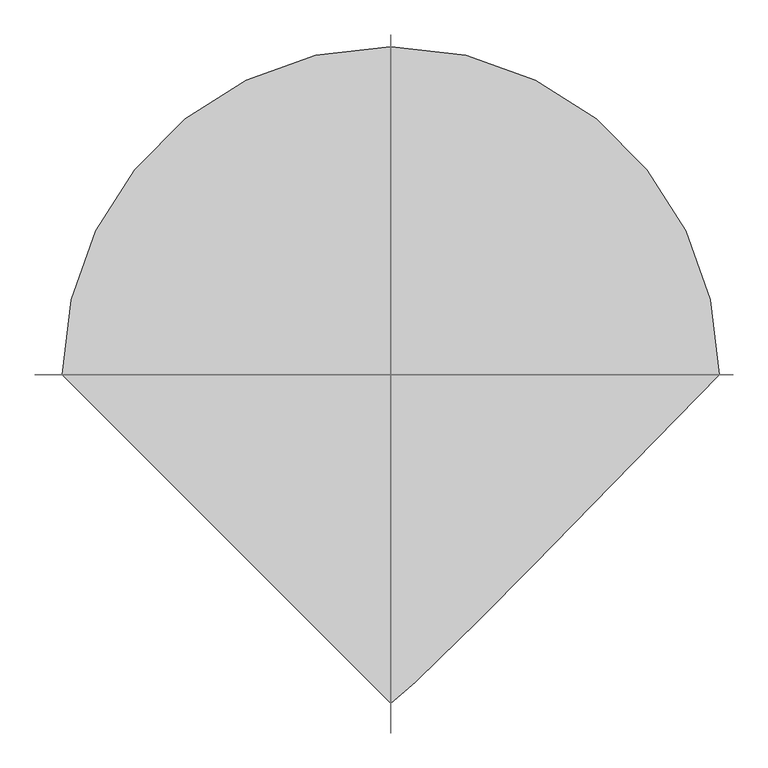
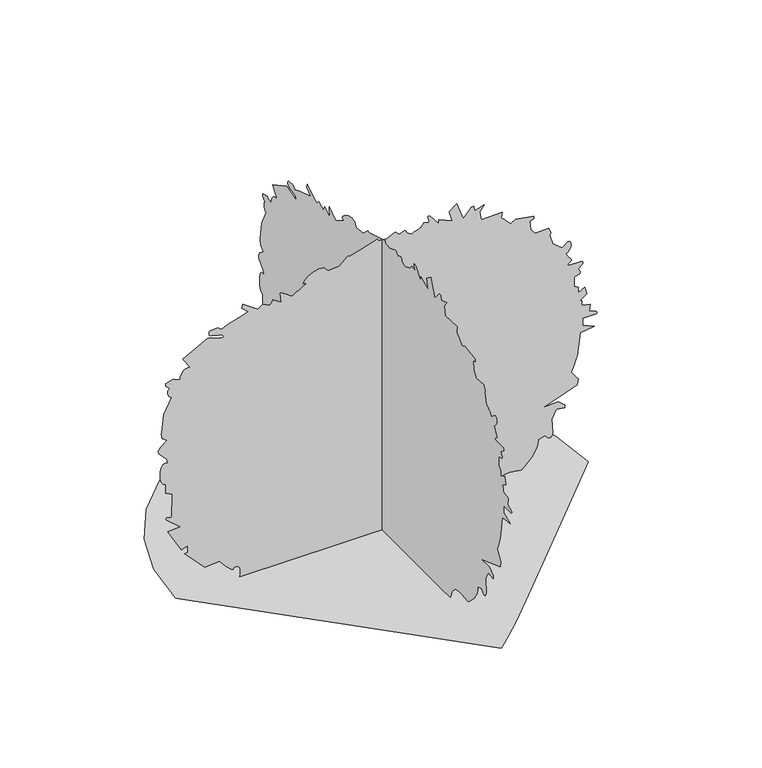
"""IFC4 building model written with IfcOpenShell, lengths in millimetres: proxy geometry, holly 26751 : holly 26751."""

from ifc_helpers import new_model, si_unit, origin, place, context, project, spatial, triangles, source, transform, mapped, element, save


def entourage_04c35473(model_context):
    return source(origin(), model_context, "Body", "Tessellation", [
        triangles([(-823.0310858, 0.0, 7.21e-05), (-801.2709314, 188.5840741, 7.21e-05), (-739.3050917, 361.7670897, 7.21e-05), (-642.0891506, 514.5912643, 7.21e-05), (-514.5912643, 642.0891506, 7.21e-05), (-361.7670897, 739.3050917, 7.21e-05), (-188.5840741, 801.2709314, 7.21e-05), (3.6e-05, 823.0310858, 7.21e-05), (188.5840741, 801.2709314, 7.21e-05), (361.7670897, 739.3050917, 7.21e-05), (514.5912643, 642.0891506, 7.21e-05), (642.0891506, 514.5912643, 7.21e-05), (739.3050917, 361.7670897, 7.21e-05), (801.2709314, 188.5838197, 7.21e-05), (823.0310858, -7.2e-05, 7.21e-05), (555.5640178, -274.3555465, 7.21e-05), (357.2763754, -476.3515926, 7.21e-05), (216.6411551, -618.0454874, 7.21e-05), (122.1254853, -711.5022102, 7.21e-05), (62.2002777, -768.7766939, 7.21e-05), (25.3349997, -801.933827, 7.21e-05), (-0.0001079, -823.0310858, 7.21e-05), (0.0, -364.688096, 1198.1839863), (0.0, -394.9268025, 1235.9816792), (0.0, -406.2653546, 1235.9816792), (0.0, -410.0448841, 1217.0841408), (0.0, -447.8426133, 1228.4226929), (0.0, -428.9450386, 1205.7430452), (0.0, -436.5040612, 1167.9452797), (0.0, -519.6585786, 1171.727389), (0.0, -515.8790491, 1149.0476686), (0.0, -517.7484844, 1147.6176687), (0.0, -521.9039357, 1143.7644882), (0.0, -527.6798913, 1138.1510954), (0.0, -534.4109121, 1131.4328281), (0.0, -541.4314502, 1124.2699659), (0.0, -548.0735593, 1117.3230789), (0.0, -553.6768147, 1111.2499758), (0.0, -572.5743894, 1122.5885279), (0.0, -644.390391, 1111.2499758), (0.0, -644.390391, 1099.9114237), (0.0, -629.2722731, 1096.1318579), (0.0, -633.0517662, 1058.334165), (0.0, -651.9493773, 1035.6544447), (0.0, -704.8677315, 1039.4340105), (0.0, -712.4267904, 1016.7569063), (0.0, -708.6472973, 1009.1953039), (0.0, -719.9858494, 967.6180452), (0.0, -726.0208735, 963.2238367), (0.0, -732.9550432, 957.9761919), (0.0, -740.1179054, 952.4085085), (0.0, -746.8488899, 947.0389961), (0.0, -752.4800869, 942.3932768), (0.0, -756.345912, 938.9998793), (0.0, -757.7835423, 937.3818821), (0.0, -780.4607191, 956.2794931), (0.0, -789.1297394, 953.9172827), (0.0, -793.4883396, 947.7375), (0.0, -794.1741262, 939.096385), (0.0, -791.8195461, 929.3580259), (0.0, -787.0672199, 919.8812788), (0.0, -780.5495945, 912.0225288), (0.0, -772.9016602, 907.1431755), (0.0, -774.118301, 904.8622828), (-2e-07, -781.5884846, 895.1949949), (-2e-07, -794.0852509, 877.4074179), (0.0, -795.5813078, 873.1249758), (0.0, -794.0014624, 870.5621235), (0.0, -782.7695171, 862.2893), (0.0, -780.9686823, 860.2395704), (0.0, -780.4607191, 858.0068579), (2e-07, -785.7515299, 855.1773067), (-2e-07, -836.9528378, 853.0538898), (0.0, -840.9380596, 850.4453281), (1e-07, -841.2580982, 846.6200529), (1e-07, -839.7290491, 843.1504246), (0.0, -822.0405212, 827.768224), (3e-07, -829.193137, 816.4016939), (5e-07, -829.9424372, 812.9472536), (7e-07, -829.5335232, 809.4446331), (7e-07, -829.7087305, 806.8944981), (6e-07, -827.806303, 805.096134), (0.0, -810.7247875, 799.7900625), (0.0, -806.9198599, 797.5295174), (0.0, -806.9198599, 759.7317518), (0.0, -822.0405212, 748.3931997), (0.0, -822.0405212, 725.7135521), (0.0, -848.4971186, 740.8341408), (0.0, -856.0561775, 710.5954342), (0.0, -829.5995075, 691.6952797), (0.0, -837.1585665, 687.9157866), (0.0, -837.1585665, 669.0181755), (0.0, -871.1767662, 661.4591892), (0.0, -867.3972731, 631.2204826), (-4e-07, -892.5458107, 622.5819111), (-3e-07, -895.9697296, 619.724382), (0.0, -897.6334362, 616.1023647), (3e-07, -893.5719835, 613.0467373), (0.0, -840.9380596, 612.3203281), (0.0, -840.9380596, 582.084165), (0.0, -886.2948841, 563.1840105), (0.0, -829.5995075, 555.6249879), (0.0, -818.258412, 461.1319184), (0.0, -815.0631128, 451.4214646), (0.0, -811.202302, 440.3089889), (0.0, -807.0646185, 428.8484965), (0.0, -803.043861, 418.0966819), (0.0, -799.5284506, 409.1101665), (0.0, -796.9122585, 402.9455718), (0.0, -795.5813078, 400.6545053), (0.0, -820.5621958, 364.3553764), (0.0, -822.0405212, 362.856776), (0.0, -818.258412, 340.1796355), (-1.2e-06, -685.9676497, 291.7393147), (0.0, -742.6629536, 294.8203221), (0.0, -767.2044062, 273.0017229), (0.0, -769.1220943, 272.1432179), (0.0, -769.1220943, 260.8046476), (0.0, -735.1038946, 264.5841771), (0.0, -716.2062836, 230.5654505), (6e-07, -720.5065298, 170.5523622), (4e-07, -718.0097345, 161.443416), (0.0, -712.4267904, 154.9702283), (1e-07, -708.1747971, 154.6016643), (1e-07, -704.4080212, 155.6534715), (1e-07, -701.0399855, 157.7794682), (0.0, -689.7471428, 170.0893091), (0.0, -663.2904728, 162.5297596), (0.0, -661.3549805, 143.989803), (0.0, -655.9651205, 127.1831253), (0.0, -637.3164768, 97.7790698), (0.0, -599.0335665, 60.4761278), (0.0, -593.0747369, 58.4339696), (0.0, -555.4065419, 64.3069578), (0.0, -530.3748576, 63.9444981), (0.0, -505.6580887, 55.865013), (0.0, -484.5938948, 35.9298222), (0.0, -470.5222973, 0.0), (1.9e-06, 527.336998, 0.3946068), (1.9e-06, 526.7324927, 3.4093656), (1.8e-06, 525.6326689, 11.1126779), (1.6e-06, 525.1043581, 21.4932261), (1.4e-06, 526.211776, 32.5396858), (1.3e-06, 530.0217905, 42.240454), (1.2e-06, 537.6011244, 48.584103), (1.1e-06, 550.0141022, 49.5597157), (1.1e-06, 552.9884482, 42.5897014), (9e-07, 560.6973527, 44.5830936), (4e-07, 583.0569617, 64.6592528), (2e-07, 594.0755116, 77.3417272), (1e-07, 602.5667084, 88.1867683), (0.0, 606.7119859, 94.4940959), (0.0, 667.1868193, 90.7143212), (0.0, 746.5618435, 173.8690929), (0.0, 735.2232914, 177.6488585), (0.0, 735.2232914, 204.1070183), (0.0, 761.6799614, 196.547487), (0.0, 814.5983156, 291.0408108), (0.0, 765.461998, 294.8203221), (-1e-07, 818.4387789, 340.9873624), (0.0, 822.1573019, 347.7386945), (-3e-07, 820.8568726, 350.2888295), (-4e-07, 818.2406805, 351.2819738), (0.0, 799.4776543, 347.7386945), (0.0, 795.6981611, 442.2317639), (0.0, 822.1573019, 457.352389), (0.0, 822.1573019, 495.1475747), (0.0, 832.8634071, 498.9677267), (1e-07, 839.8280983, 508.9931322), (2e-07, 843.5822296, 523.0672731), (5e-07, 843.58986, 554.7486969), (7e-07, 840.9076109, 568.0481031), (9e-07, 837.1458492, 576.780637), (6e-07, 835.3424709, 579.5238198), (4e-07, 832.4240444, 581.3678933), (1e-07, 824.7836678, 582.9223406), (0.0, 814.5983156, 582.084165), (0.0, 818.9670897, 599.2621862), (0.0, 850.1633686, 632.368523), (0.0, 852.289329, 643.412471), (0.0, 843.1225193, 657.5323214), (0.0, 818.3778088, 676.5772345), (0.0, 819.0966602, 678.065661), (0.0, 834.2578714, 690.2068531), (0.0, 837.2754198, 691.6952797), (0.0, 841.0549129, 714.375), (0.0, 838.9950096, 718.3525915), (0.0, 829.7163609, 789.9704584), (0.0, 799.4776543, 854.2273647), (0.0, 805.1469303, 855.9037886), (0.0, 809.7265926, 860.3360762), (0.0, 812.954884, 866.6098938), (0.0, 814.5627073, 873.8234797), (0.0, 814.2909216, 881.0700577), (0.0, 811.8703571, 887.4378376), (0.0, 807.0392567, 892.0251303), (0.0, 807.4354534, 892.8607624), (0.0, 812.0837162, 897.9737497), (0.0, 820.8492422, 906.3049999), (0.0, 822.1573019, 907.1431755), (0.0, 822.1573019, 918.4817276), (0.0, 791.9185953, 926.0407866), (0.0, 790.6511581, 925.0044399), (0.0, 777.4609749, 918.7560568), (0.0, 765.461998, 914.7022345), (0.0, 764.4104633, 924.481216), (0.0, 761.392915, 934.0036726), (0.0, 756.6100674, 942.5457384), (0.0, 750.2651785, 949.3884893), (0.0, 742.5613609, 953.8080597), (0.0, 733.6992565, 955.0856707), (0.0, 723.8821959, 952.5), (0.0, 754.1209024, 997.8567518), (0.0, 655.8482672, 1050.775106), (7e-07, 598.9294304, 1033.6808733), (5e-07, 592.5108541, 1034.3742903), (5e-07, 591.6802726, 1035.5045992), (4e-07, 591.6421935, 1037.1784796), (3e-07, 592.2771838, 1039.2003038), (2e-07, 595.0864237, 1043.5360857), (0.0, 599.1504198, 1046.9930695), (0.0, 613.793494, 1050.1477461), (0.0, 641.0578909, 1056.558692), (0.0, 644.5071716, 1058.334165), (1e-07, 646.8948166, 1060.1705355), (1e-07, 648.7185425, 1062.5454632), (1e-07, 649.9529875, 1065.3064138), (1e-07, 650.5574564, 1068.3061581), (0.0, 650.5041166, 1071.3923069), (0.0, 649.7573599, 1074.4174129), (0.0, 648.2892809, 1077.2317034), (-2e-07, 645.2513849, 1079.2662449), (0.0, 614.2710085, 1081.0112692), (0.0, 603.3617543, 1070.5744062), (0.0, 602.9299493, 1069.6727171), (0.0, 567.8931707, 1083.2083735), (0.0, 547.3801423, 1090.3508154), (0.0, 493.3187983, 1107.47041), (0.0, 519.7754319, 1130.1475868), (0.0, 515.9959024, 1145.2681755), (0.0, 455.5210327, 1103.6909168), (0.0, 436.6209146, 1118.8089621), (0.0, 406.382208, 1103.6909168), (0.0, 405.4525772, 1104.4097683), (0.0, 396.018996, 1119.5709795), (0.0, 395.0436559, 1122.5885279), (0.0, 361.0254198, 1099.9114237), (0.0, 365.1427557, 1139.9113077), (0.0, 364.8049493, 1141.4886824), (0.0, 342.607903, 1128.2831657), (0.0, 319.4481611, 1111.2499758), (0.0, 309.9866747, 1116.2283783), (0.0, 299.4278897, 1122.1567228), (0.0, 288.7040166, 1128.4457285), (0.0, 278.7446681, 1134.4934698), (0.0, 270.4795113, 1139.7106659), (0.0, 264.8381769, 1143.5003328), (0.0, 262.752839, 1145.2681755), (0.0, 273.3471778, 1149.5912401), (0.0, 269.0418629, 1159.9925674), (0.0, 254.1727123, 1172.6036436), (0.0, 233.0803043, 1183.5662739), (0.0, 210.0991489, 1189.0196474), (0.0, 189.5657729, 1185.1004826), (0.0, 175.8177748, 1167.9452797), (0.0, 130.4607414, 1171.727389), (0.0, 96.4430322, 1201.9634794), (0.0, 95.7204019, 1201.8238077), (0.0, 89.6495515, 1198.8037886), (0.0, 88.8834827, 1198.1839863), (0.0, 39.7464248, 1213.3046476), (0.0, -20.7297008, 1232.2022587), (0.0, -21.3109812, 1231.442712), (0.0, -21.9957141, 1230.3632721), (0.0, -22.7131871, 1229.0906754), (0.0, -23.3937551, 1227.7547104), (0.0, -23.9666262, 1226.4821136), (0.0, -24.3619509, 1225.4026737), (0.0, -24.5094506, 1224.6431271), (0.0, -58.527187, 1220.8637066), (0.0, -88.228163, 1235.3035229), (0.0, -92.5451506, 1235.9816792), (-1e-07, -95.4963785, 1234.686264), (0.0, -109.5573117, 1221.6231079), (0.0, -111.4440243, 1220.8637066), (0.0, -122.4526365, 1227.7801449), (0.0, -128.2821862, 1229.7790054), (0.0, -133.4833494, 1229.5072197), (0.0, -137.0317248, 1225.6972778), (0.0, -137.9024383, 1217.0841408), (0.0, -140.9202138, 1215.7049372), (0.0, -144.3867991, 1213.9269207), (0.0, -147.9687116, 1211.9380886), (0.0, -151.3339586, 1209.9340685), (0.0, -154.1492937, 1208.1052557), (0.0, -156.0827331, 1206.6447344), (0.0, -156.801312, 1205.7430452), (0.0, -162.3971732, 1208.1433348), (0.0, -169.0263289, 1210.9119158), (0.0, -176.0290991, 1213.7770752), (0.0, -182.746894, 1216.4745123), (0.0, -188.5205787, 1218.7325867), (0.0, -192.691, 1220.2871429), (0.0, -194.5987869, 1220.8637066), (0.0, -205.4400219, 1235.8141022), (0.0, -205.9381202, 1235.9816792), (0.0, -208.316318, 1235.3645657), (0.0, -227.1496525, 1232.3444012), (0.0, -228.6167504, 1232.2022587), (1e-07, -223.3642912, 1249.3599323), (1e-07, -222.9002389, 1253.4188416), (1e-07, -223.3033211, 1256.642046), (0.0, -224.8369848, 1258.6613995), (-3e-07, -231.8636453, 1254.2900093), (0.0, -264.139673, 1215.5067661), (0.0, -266.4129717, 1213.3046476), (0.0, -266.4129717, 1228.4226929), (0.0, -319.3313441, 1205.7430452), (0.0, -307.9927557, 1247.3202312), (0.0, -338.2289188, 1269.9999516), (325.0107576, 3.63e-05, 1198.1839863), (355.2494642, 3.85e-05, 1235.9816792), (366.5880163, 3.85e-05, 1235.9816792), (370.3675458, 3.74e-05, 1217.0841408), (408.165275, 3.81e-05, 1228.4226929), (389.2677003, 3.67e-05, 1205.7430452), (396.8267229, 3.44e-05, 1167.9452797), (479.9812403, 3.47e-05, 1171.727389), (476.2017108, 3.33e-05, 1149.0476686), (478.0711461, 3.32e-05, 1147.6176687), (482.2265974, 3.3e-05, 1143.7644882), (488.002553, 3.27e-05, 1138.1510954), (494.7335738, 3.23e-05, 1131.4328281), (501.7515684, 3.18e-05, 1124.2699659), (508.396221, 3.14e-05, 1117.3230789), (513.9994763, 3.11e-05, 1111.2499758), (532.897051, 3.17e-05, 1122.5885279), (604.7130163, 3.11e-05, 1111.2499758), (604.7130163, 3.04e-05, 1099.9114237), (589.5949347, 3.02e-05, 1096.1318579), (593.3744642, 2.79e-05, 1058.334165), (612.2720753, 2.66e-05, 1035.6544447), (665.187886, 2.68e-05, 1039.4340105), (672.7494884, 2.54e-05, 1016.7569063), (668.9699226, 2.5e-05, 1009.1953039), (680.3084747, 2.25e-05, 967.6180452), (686.3434988, 2.22e-05, 963.2238367), (693.2777412, 2.19e-05, 957.9761919), (700.4405308, 2.16e-05, 952.4085085), (707.1715153, 2.13e-05, 947.0389961), (712.8027122, 2.1e-05, 942.3932768), (716.66861, 2.08e-05, 938.9998793), (718.1062403, 2.07e-05, 937.3818821), (740.7833445, 2.18e-05, 956.2794931), (749.4523647, 2.17e-05, 953.9172827), (753.8110376, 2.13e-05, 947.7375), (754.4942808, 2.08e-05, 939.096385), (752.1422441, 2.02e-05, 929.3580259), (747.3899179, 1.97e-05, 919.8812788), (740.8722198, 1.92e-05, 912.0225288), (733.2242855, 1.89e-05, 907.1431755), (734.440999, 1.87e-05, 904.8622828), (741.9111099, 1.8e-05, 895.1949949), (754.4078762, 1.69e-05, 877.4074179), (755.9040058, 1.69e-05, 873.1249758), (754.3240877, 1.68e-05, 870.5621235), (743.0922152, 1.62e-05, 862.2893), (741.2913803, 1.61e-05, 860.2395704), (740.7833445, 1.6e-05, 858.0068579), (746.0741552, 1.6e-05, 855.1773067), (797.2754631, 1.54e-05, 853.0538898), (801.2607576, 1.55e-05, 850.4453281), (801.5807962, 1.54e-05, 846.6200529), (800.0516745, 1.52e-05, 843.1504246), (782.3606031, 1.42e-05, 827.768224), (789.5157623, 1.38e-05, 816.4016939), (790.2650625, 1.38e-05, 812.9472536), (789.8561485, 1.38e-05, 809.4446331), (790.0314285, 1.36e-05, 806.8944981), (788.1289284, 1.34e-05, 805.096134), (771.0474855, 1.25e-05, 799.7900625), (767.2425579, 1.24e-05, 797.5295174), (767.2425579, 1.01e-05, 759.7317518), (782.3606031, 9.4e-06, 748.3931997), (782.3606031, 8.1e-06, 725.7135521), (808.8198166, 9e-06, 740.8341408), (816.3788029, 7.2e-06, 710.5954342), (789.9222055, 6.1e-06, 691.6952797), (797.4812645, 5.8e-06, 687.9157866), (797.4812645, 4.7e-06, 669.0181755), (831.4994642, 4.3e-06, 661.4591892), (827.7198984, 2.5e-06, 631.2204826), (852.8684361, 1.6e-06, 622.5819111), (856.292355, 1.5e-06, 619.724382), (857.9560616, 1.6e-06, 616.1023647), (853.8946089, 1.7e-06, 613.0467373), (801.2607576, 1.3e-06, 612.3203281), (801.2607576, -5e-07, 582.084165), (846.6175095, -1.6e-06, 563.1840105), (789.9222055, -2e-06, 555.6249879), (778.58111, -7.7e-06, 461.1319184), (775.3857382, -8.3e-06, 451.4214646), (771.525, -8.9e-06, 440.3089889), (767.3873165, -9.6e-06, 428.8484965), (763.3664864, -1.02e-05, 418.0966819), (759.8511486, -1.08e-05, 409.1101665), (757.2349566, -1.11e-05, 402.9455718), (755.9040058, -1.13e-05, 400.6545053), (780.8823503, -1.34e-05, 364.3553764), (782.3606031, -1.35e-05, 362.856776), (778.58111, -1.49e-05, 340.1796355), (646.290275, -1.9e-05, 291.7393147), (702.9855789, -1.76e-05, 294.8203221), (727.5271042, -1.89e-05, 273.0017229), (729.4447924, -1.89e-05, 272.1432179), (729.4447924, -1.96e-05, 260.8046476), (695.4265926, -1.94e-05, 264.5841771), (676.5289816, -2.14e-05, 230.5654505), (680.8292278, -2.44e-05, 170.5523622), (678.3323599, -2.51e-05, 161.4436704), (672.7494884, -2.59e-05, 154.9702283), (668.4974951, -2.59e-05, 154.6016643), (664.7306465, -2.58e-05, 155.6534715), (661.3626108, -2.56e-05, 157.7794682), (650.0697681, -2.5e-05, 170.0893091), (623.6106274, -2.55e-05, 162.5297596), (621.675135, -2.66e-05, 143.989803), (616.2852751, -2.76e-05, 127.1833797), (597.6391022, -2.93e-05, 97.7790698), (559.3562282, -3.16e-05, 60.4761278), (553.3948551, -3.17e-05, 58.4342239), (515.7292036, -3.13e-05, 64.3069578), (490.6975193, -3.14e-05, 63.9444981), (465.9807504, -3.18e-05, 55.8652674), (444.9165565, -3.3e-05, 35.9298222), (430.844959, -3.52e-05, 5e-05), (-567.0143363, -3.32e-05, 0.3946575), (-566.409831, -3.31e-05, 3.4094164), (-565.3100072, -3.27e-05, 11.1127279), (-564.7816964, -3.23e-05, 21.4932761), (-565.8891143, -3.18e-05, 32.5396858), (-569.6991288, -3.14e-05, 42.240454), (-577.2784627, -3.11e-05, 48.584103), (-589.6914405, -3.11e-05, 49.5597157), (-592.6657866, -3.16e-05, 42.5897014), (-600.374691, -3.16e-05, 44.5830936), (-622.7343, -3.09e-05, 64.6592528), (-633.7528135, -3.03e-05, 77.3417272), (-642.244083, -2.98e-05, 88.1867683), (-646.3893242, -2.95e-05, 94.4940959), (-706.8641939, -2.98e-05, 90.7143212), (-786.2392181, -2.48e-05, 173.8690929), (-774.900666, -2.46e-05, 177.6488585), (-774.900666, -2.3e-05, 204.1072726), (-801.3598068, -2.35e-05, 196.5477413), (-854.2756176, -1.78e-05, 291.0408108), (-805.1393, -1.76e-05, 294.8203221), (-858.1160809, -1.5e-05, 340.9873624), (-861.8346766, -1.44e-05, 347.7386945), (-860.5341745, -1.46e-05, 350.2888295), (-857.9179825, -1.46e-05, 351.2819738), (-839.1550289, -1.44e-05, 347.7386945), (-835.3754631, -8.8e-06, 442.2317639), (-861.8346766, -7.9e-06, 457.352389), (-861.8346766, -5.7e-06, 495.1475747), (-872.5433252, -5.4e-06, 498.9677267), (-879.5054729, -4.7e-06, 508.9931322), (-883.2595316, -3.8e-06, 523.0672731), (-883.2671619, -1.6e-06, 554.7486969), (-880.5874563, -6e-07, 568.0481031), (-876.8257673, 2e-07, 576.780637), (-875.0197729, 0.0, 579.5238198), (-872.1013464, -1e-07, 581.3678933), (-864.4610424, -3e-07, 582.9223406), (-854.2756176, -5e-07, 582.084165), (-858.6443916, 6e-07, 599.2621862), (-889.8406706, 2.5e-06, 632.368523), (-891.9667036, 3.2e-06, 643.412471), (-882.8023647, 4e-06, 657.5323214), (-858.0551834, 5.2e-06, 676.5772345), (-858.7739622, 5.2e-06, 678.065661), (-873.9352461, 6e-06, 690.2068531), (-876.9527218, 6.1e-06, 691.6952797), (-880.734831, 7.4e-06, 714.375), (-878.6723116, 7.7e-06, 718.3525915), (-869.3937355, 1.19e-05, 789.9704584), (-839.1550289, 1.57e-05, 854.2273647), (-844.824305, 1.58e-05, 855.9037886), (-849.4064381, 1.61e-05, 860.3360762), (-852.6322586, 1.65e-05, 866.6098938), (-854.240082, 1.69e-05, 873.8234797), (-853.9682962, 1.73e-05, 881.0700577), (-851.5476591, 1.77e-05, 887.4378376), (-846.7165586, 1.8e-05, 892.0225868), (-847.1128281, 1.81e-05, 892.8607624), (-851.7610182, 1.84e-05, 897.9737497), (-860.5265442, 1.89e-05, 906.3049999), (-861.8346766, 1.89e-05, 907.1431755), (-861.8346766, 1.96e-05, 918.4817276), (-831.59597, 2e-05, 926.0407866), (-830.3285328, 2e-05, 925.0044399), (-817.1382769, 1.96e-05, 918.7560568), (-805.1393, 1.94e-05, 914.7022345), (-804.0877653, 1.99e-05, 924.481216), (-801.0702169, 2.05e-05, 934.0036726), (-796.287442, 2.1e-05, 942.5457384), (-789.9424805, 2.14e-05, 949.3884893), (-782.2386629, 2.17e-05, 953.8080597), (-773.3766312, 2.18e-05, 955.0856707), (-763.5620413, 2.16e-05, 952.5), (-793.7982044, 2.43e-05, 997.8567518), (-695.5256418, 2.75e-05, 1050.775106), (-638.606805, 2.72e-05, 1033.6808733), (-632.1882288, 2.7e-05, 1034.3742903), (-631.3576109, 2.7e-05, 1035.5045992), (-631.3195318, 2.71e-05, 1037.1784796), (-631.9545221, 2.71e-05, 1039.2003038), (-634.7637257, 2.72e-05, 1043.5360857), (-638.8277218, 2.72e-05, 1046.9930695), (-653.4708687, 2.74e-05, 1050.1477461), (-680.7351929, 2.78e-05, 1056.558692), (-684.1870897, 2.79e-05, 1058.334165), (-686.5721186, 2.81e-05, 1060.1705355), (-688.3983879, 2.83e-05, 1062.5454632), (-689.6302895, 2.84e-05, 1065.3064138), (-690.234831, 2.86e-05, 1068.3061581), (-690.1814913, 2.87e-05, 1071.3923069), (-689.4347345, 2.89e-05, 1074.4174129), (-687.9665829, 2.9e-05, 1077.2317034), (-684.9287596, 2.9e-05, 1079.2637741), (-653.9483831, 2.93e-05, 1081.0112692), (-643.0390926, 2.86e-05, 1070.5744062), (-642.609831, 2.86e-05, 1069.6727171), (-607.5705091, 2.94e-05, 1083.2083735), (-587.0574806, 2.98e-05, 1090.3508154), (-532.9961366, 3.08e-05, 1107.47041), (-559.4527702, 3.22e-05, 1130.1475868), (-555.6732408, 3.31e-05, 1145.2681755), (-495.198371, 3.06e-05, 1103.6909168), (-476.2982529, 3.15e-05, 1118.8089621), (-446.0620897, 3.06e-05, 1103.6909168), (-445.1299155, 3.07e-05, 1104.4097683), (-435.6963344, 3.16e-05, 1119.5709795), (-434.7209942, 3.17e-05, 1122.5885279), (-400.7027581, 3.04e-05, 1099.9114237), (-404.820094, 3.28e-05, 1139.9113077), (-404.484831, 3.29e-05, 1141.4886824), (-382.2852413, 3.21e-05, 1128.2831657), (-359.1254994, 3.11e-05, 1111.2499758), (-349.664013, 3.14e-05, 1116.2283783), (-339.1052098, 3.17e-05, 1122.1567228), (-328.3813368, 3.21e-05, 1128.4457285), (-318.4220246, 3.25e-05, 1134.4934698), (-310.1568315, 3.28e-05, 1139.7106659), (-304.5180405, 3.3e-05, 1143.5003328), (-302.4301774, 3.31e-05, 1145.2681755), (-313.024498, 3.34e-05, 1149.5912401), (-308.7192012, 3.4e-05, 1159.990024), (-293.8500506, 3.47e-05, 1172.6036436), (-272.7578969, 3.54e-05, 1183.5662739), (-249.7767416, 3.57e-05, 1189.0196474), (-229.2433655, 3.55e-05, 1185.1004826), (-215.4953675, 3.44e-05, 1167.9452797), (-170.1383431, 3.47e-05, 1171.727389), (-136.1206249, 3.65e-05, 1201.9634794), (-135.3979945, 3.65e-05, 1201.8238077), (-129.3271442, 3.63e-05, 1198.8037886), (-128.5610754, 3.63e-05, 1198.1839863), (-79.424022, 3.72e-05, 1213.3046476), (-18.9479168, 3.83e-05, 1232.2022587), (-18.3666376, 3.82e-05, 1231.442712), (-17.6819047, 3.82e-05, 1230.3632721), (-16.9644305, 3.81e-05, 1229.0906754), (-16.2838637, 3.8e-05, 1227.7547104), (-15.7109914, 3.79e-05, 1226.4821136), (-15.3156656, 3.79e-05, 1225.4026737), (-15.1681682, 3.78e-05, 1224.6431271), (18.8496693, 3.76e-05, 1220.8637066), (48.5505749, 3.84e-05, 1235.3035229), (52.8675579, 3.85e-05, 1235.9816792), (55.8187858, 3.84e-05, 1234.686264), (69.8797145, 3.76e-05, 1221.6231079), (71.7664271, 3.76e-05, 1220.8637066), (82.7750438, 3.8e-05, 1227.7801449), (88.6045935, 3.81e-05, 1229.7790054), (93.8057568, 3.81e-05, 1229.5072197), (97.3541321, 3.79e-05, 1225.6972778), (98.2248457, 3.74e-05, 1217.0841408), (101.2426211, 3.73e-05, 1215.7049372), (104.7092064, 3.72e-05, 1213.9269207), (108.291119, 3.71e-05, 1211.9380886), (111.6563659, 3.7e-05, 1209.9340685), (114.471701, 3.68e-05, 1208.1052557), (116.4051495, 3.68e-05, 1206.6447344), (117.1234559, 3.67e-05, 1205.7430452), (122.7195896, 3.68e-05, 1208.1433348), (129.3487362, 3.7e-05, 1210.9119158), (136.3515156, 3.72e-05, 1213.7770752), (143.0693014, 3.73e-05, 1216.4745123), (148.8427226, 3.75e-05, 1218.7325867), (153.013153, 3.76e-05, 1220.2871429), (154.9211942, 3.76e-05, 1220.8637066), (165.7624293, 3.85e-05, 1235.8141022), (166.2605275, 3.85e-05, 1235.9816792), (168.6387254, 3.85e-05, 1235.3645657), (187.4720598, 3.83e-05, 1232.3444012), (188.9389034, 3.83e-05, 1232.2022587), (183.6866986, 3.94e-05, 1249.3599323), (183.2226462, 3.96e-05, 1253.4188416), (183.6257285, 3.98e-05, 1256.642046), (185.1593921, 3.99e-05, 1258.6613995), (192.1860526, 3.93e-05, 1254.2900093), (224.4613173, 3.72e-05, 1215.5067661), (226.7366508, 3.72e-05, 1213.3046476), (226.7366508, 3.81e-05, 1228.4226929), (279.6539876, 3.67e-05, 1205.7430452), (268.3128921, 3.92e-05, 1247.3202312), (298.5515805, 4.05e-05, 1269.9999516)], [[22, 21, 1], [21, 20, 1], [20, 19, 1], [19, 18, 1], [18, 17, 1], [1, 17, 2], [2, 17, 3], [3, 17, 4], [17, 16, 4], [4, 16, 5], [5, 16, 6], [6, 16, 7], [7, 16, 8], [8, 16, 9], [9, 16, 10], [10, 16, 11], [11, 16, 12], [16, 15, 12], [15, 14, 12], [14, 13, 12], [101, 100, 102], [27, 26, 28], [154, 153, 155], [158, 157, 159], [317, 316, 318], [240, 239, 241], [239, 238, 241], [320, 319, 23], [319, 318, 23], [246, 245, 247], [88, 87, 89], [157, 156, 159], [30, 29, 31], [139, 138, 140], [249, 248, 250], [140, 138, 141], [118, 117, 119], [117, 116, 119], [213, 212, 214], [141, 138, 142], [259, 258, 260], [313, 312, 314], [312, 311, 314], [311, 310, 314], [93, 92, 94], [142, 138, 143], [147, 146, 148], [40, 39, 41], [41, 39, 42], [25, 24, 26], [97, 96, 98], [201, 200, 202], [200, 199, 202], [199, 198, 202], [202, 198, 203], [198, 197, 203], [45, 44, 46], [46, 44, 47], [310, 309, 314], [260, 258, 261], [203, 197, 204], [197, 196, 204], [138, 137, 143], [272, 271, 273], [273, 271, 274], [274, 271, 275], [275, 271, 276], [276, 271, 277], [277, 271, 278], [278, 271, 279], [96, 95, 98], [95, 94, 98], [98, 94, 99], [94, 92, 99], [248, 247, 250], [143, 137, 144], [24, 23, 26], [242, 241, 243], [89, 87, 90], [250, 247, 251], [116, 115, 119], [119, 115, 120], [115, 114, 120], [91, 90, 92], [113, 112, 114], [112, 111, 114], [111, 110, 114], [166, 165, 167], [42, 39, 43], [39, 38, 43], [245, 244, 247], [161, 160, 162], [162, 160, 163], [163, 160, 164], [56, 55, 57], [57, 55, 58], [58, 55, 59], [59, 55, 60], [60, 55, 61], [61, 55, 62], [62, 55, 63], [185, 184, 186], [86, 85, 87], [267, 266, 268], [268, 266, 269], [269, 266, 270], [74, 73, 75], [75, 73, 76], [73, 72, 76], [76, 72, 77], [67, 66, 68], [81, 80, 82], [47, 44, 48], [160, 159, 164], [26, 23, 28], [28, 23, 29], [155, 153, 156], [68, 66, 69], [214, 212, 215], [66, 65, 69], [261, 258, 262], [123, 122, 124], [124, 122, 125], [125, 122, 126], [122, 121, 126], [126, 121, 127], [288, 287, 289], [289, 287, 290], [287, 286, 290], [286, 285, 290], [180, 179, 181], [181, 179, 182], [179, 178, 182], [137, 136, 144], [244, 243, 247], [69, 65, 70], [186, 184, 187], [184, 183, 187], [204, 196, 205], [153, 152, 156], [144, 136, 145], [264, 263, 265], [263, 262, 265], [262, 258, 265], [121, 120, 127], [120, 114, 127], [127, 114, 128], [148, 146, 149], [168, 167, 169], [169, 167, 170], [80, 79, 82], [79, 78, 82], [82, 78, 83], [78, 77, 83], [77, 72, 83], [83, 72, 84], [72, 71, 84], [314, 309, 315], [306, 305, 307], [305, 304, 307], [282, 281, 283], [281, 280, 283], [283, 280, 284], [65, 64, 70], [156, 152, 159], [170, 167, 171], [171, 167, 172], [172, 167, 173], [173, 167, 174], [174, 167, 175], [175, 167, 176], [176, 167, 177], [167, 165, 177], [164, 159, 165], [307, 304, 308], [231, 230, 232], [230, 229, 232], [229, 228, 232], [228, 227, 232], [227, 226, 232], [226, 225, 232], [225, 224, 232], [224, 223, 232], [232, 223, 233], [223, 222, 233], [233, 222, 234], [234, 222, 235], [222, 221, 235], [221, 220, 235], [235, 220, 236], [220, 219, 236], [219, 218, 236], [236, 218, 237], [218, 217, 237], [237, 217, 238], [133, 132, 134], [132, 131, 134], [190, 189, 191], [191, 189, 192], [192, 189, 193], [193, 189, 194], [194, 189, 195], [195, 189, 196], [196, 189, 205], [187, 183, 188], [215, 212, 216], [159, 152, 165], [131, 130, 134], [130, 129, 134], [129, 128, 134], [134, 128, 135], [128, 114, 135], [135, 114, 136], [136, 114, 145], [114, 110, 145], [110, 109, 145], [109, 108, 145], [108, 107, 145], [107, 106, 145], [106, 105, 145], [105, 104, 145], [104, 103, 145], [103, 102, 145], [102, 100, 145], [100, 99, 145], [99, 92, 145], [92, 90, 145], [90, 87, 145], [87, 85, 145], [85, 84, 145], [84, 71, 145], [71, 70, 145], [70, 64, 145], [64, 63, 145], [63, 55, 145], [55, 54, 145], [54, 53, 145], [53, 52, 145], [52, 51, 145], [51, 50, 145], [50, 49, 145], [49, 48, 145], [48, 44, 145], [44, 43, 145], [43, 38, 145], [38, 37, 145], [37, 36, 145], [36, 35, 145], [35, 34, 145], [34, 33, 145], [33, 32, 145], [32, 31, 145], [31, 29, 145], [29, 23, 145], [23, 318, 145], [318, 316, 145], [316, 315, 145], [315, 309, 145], [309, 308, 145], [308, 304, 145], [304, 303, 145], [303, 302, 145], [302, 301, 145], [301, 300, 145], [300, 299, 145], [299, 298, 145], [298, 297, 145], [297, 296, 145], [296, 295, 145], [295, 294, 145], [294, 293, 145], [293, 292, 145], [292, 291, 145], [291, 290, 145], [290, 285, 145], [285, 284, 145], [284, 280, 145], [280, 279, 145], [279, 271, 145], [271, 270, 145], [270, 266, 145], [266, 265, 145], [265, 258, 145], [258, 257, 145], [257, 256, 145], [256, 255, 145], [255, 254, 145], [254, 253, 145], [253, 252, 145], [252, 251, 145], [251, 247, 145], [247, 243, 145], [243, 241, 145], [145, 241, 146], [146, 241, 149], [149, 241, 150], [150, 241, 151], [151, 241, 152], [152, 241, 165], [165, 241, 177], [177, 241, 178], [178, 241, 182], [241, 238, 182], [238, 217, 182], [217, 216, 182], [216, 212, 182], [182, 212, 183], [183, 212, 188], [188, 212, 189], [189, 212, 205], [205, 212, 206], [206, 212, 207], [207, 212, 208], [208, 212, 209], [212, 211, 209], [211, 210, 209], [399, 398, 400], [325, 324, 326], [452, 451, 453], [456, 455, 457], [615, 614, 616], [538, 537, 539], [537, 536, 539], [618, 617, 321], [617, 616, 321], [544, 543, 545], [386, 385, 387], [455, 454, 457], [328, 327, 329], [437, 436, 438], [547, 546, 548], [438, 436, 439], [416, 415, 417], [415, 414, 417], [511, 510, 512], [439, 436, 440], [557, 556, 558], [611, 610, 612], [610, 609, 612], [609, 608, 612], [391, 390, 392], [440, 436, 441], [445, 444, 446], [338, 337, 339], [339, 337, 340], [323, 322, 324], [395, 394, 396], [499, 498, 500], [498, 497, 500], [497, 496, 500], [500, 496, 501], [496, 495, 501], [343, 342, 344], [344, 342, 345], [608, 607, 612], [558, 556, 559], [501, 495, 502], [495, 494, 502], [436, 435, 441], [570, 569, 571], [571, 569, 572], [572, 569, 573], [573, 569, 574], [574, 569, 575], [575, 569, 576], [576, 569, 577], [394, 393, 396], [393, 392, 396], [396, 392, 397], [392, 390, 397], [546, 545, 548], [441, 435, 442], [322, 321, 324], [540, 539, 541], [387, 385, 388], [548, 545, 549], [414, 413, 417], [417, 413, 418], [413, 412, 418], [389, 388, 390], [411, 410, 412], [410, 409, 412], [409, 408, 412], [464, 463, 465], [340, 337, 341], [337, 336, 341], [543, 542, 545], [459, 458, 460], [460, 458, 461], [461, 458, 462], [354, 353, 355], [355, 353, 356], [356, 353, 357], [357, 353, 358], [358, 353, 359], [359, 353, 360], [360, 353, 361], [483, 482, 484], [384, 383, 385], [565, 564, 566], [566, 564, 567], [567, 564, 568], [372, 371, 373], [373, 371, 374], [371, 370, 374], [374, 370, 375], [365, 364, 366], [379, 378, 380], [345, 342, 346], [458, 457, 462], [324, 321, 326], [326, 321, 327], [453, 451, 454], [366, 364, 367], [512, 510, 513], [364, 363, 367], [559, 556, 560], [421, 420, 422], [422, 420, 423], [423, 420, 424], [420, 419, 424], [424, 419, 425], [586, 585, 587], [587, 585, 588], [585, 584, 588], [584, 583, 588], [478, 477, 479], [479, 477, 480], [477, 476, 480], [435, 434, 442], [542, 541, 545], [367, 363, 368], [484, 482, 485], [482, 481, 485], [502, 494, 503], [451, 450, 454], [442, 434, 443], [562, 561, 563], [561, 560, 563], [560, 556, 563], [419, 418, 425], [418, 412, 425], [425, 412, 426], [446, 444, 447], [466, 465, 467], [467, 465, 468], [378, 377, 380], [377, 376, 380], [380, 376, 381], [376, 375, 381], [375, 370, 381], [381, 370, 382], [370, 369, 382], [612, 607, 613], [604, 603, 605], [603, 602, 605], [580, 579, 581], [579, 578, 581], [581, 578, 582], [363, 362, 368], [454, 450, 457], [468, 465, 469], [469, 465, 470], [470, 465, 471], [471, 465, 472], [472, 465, 473], [473, 465, 474], [474, 465, 475], [465, 463, 475], [462, 457, 463], [605, 602, 606], [529, 528, 530], [528, 527, 530], [527, 526, 530], [526, 525, 530], [525, 524, 530], [524, 523, 530], [523, 522, 530], [522, 521, 530], [530, 521, 531], [521, 520, 531], [531, 520, 532], [532, 520, 533], [520, 519, 533], [519, 518, 533], [533, 518, 534], [518, 517, 534], [517, 516, 534], [534, 516, 535], [516, 515, 535], [535, 515, 536], [431, 430, 432], [430, 429, 432], [488, 487, 489], [489, 487, 490], [490, 487, 491], [491, 487, 492], [492, 487, 493], [493, 487, 494], [494, 487, 503], [485, 481, 486], [513, 510, 514], [457, 450, 463], [429, 428, 432], [428, 427, 432], [427, 426, 432], [432, 426, 433], [426, 412, 433], [433, 412, 434], [434, 412, 443], [412, 408, 443], [408, 407, 443], [407, 406, 443], [406, 405, 443], [405, 404, 443], [404, 403, 443], [403, 402, 443], [402, 401, 443], [401, 400, 443], [400, 398, 443], [398, 397, 443], [397, 390, 443], [390, 388, 443], [388, 385, 443], [385, 383, 443], [383, 382, 443], [382, 369, 443], [369, 368, 443], [368, 362, 443], [362, 361, 443], [361, 353, 443], [353, 352, 443], [352, 351, 443], [351, 350, 443], [350, 349, 443], [349, 348, 443], [348, 347, 443], [347, 346, 443], [346, 342, 443], [342, 341, 443], [341, 336, 443], [336, 335, 443], [335, 334, 443], [334, 333, 443], [333, 332, 443], [332, 331, 443], [331, 330, 443], [330, 329, 443], [329, 327, 443], [327, 321, 443], [321, 616, 443], [616, 614, 443], [614, 613, 443], [613, 607, 443], [607, 606, 443], [606, 602, 443], [602, 601, 443], [601, 600, 443], [600, 599, 443], [599, 598, 443], [598, 597, 443], [597, 596, 443], [596, 595, 443], [595, 594, 443], [594, 593, 443], [593, 592, 443], [592, 591, 443], [591, 590, 443], [590, 589, 443], [589, 588, 443], [588, 583, 443], [583, 582, 443], [582, 578, 443], [578, 577, 443], [577, 569, 443], [569, 568, 443], [568, 564, 443], [564, 563, 443], [563, 556, 443], [556, 555, 443], [555, 554, 443], [554, 553, 443], [553, 552, 443], [552, 551, 443], [551, 550, 443], [550, 549, 443], [549, 545, 443], [545, 541, 443], [541, 539, 443], [443, 539, 444], [444, 539, 447], [447, 539, 448], [448, 539, 449], [449, 539, 450], [450, 539, 463], [463, 539, 475], [475, 539, 476], [476, 539, 480], [539, 536, 480], [536, 515, 480], [515, 514, 480], [514, 510, 480], [480, 510, 481], [481, 510, 486], [486, 510, 487], [487, 510, 503], [503, 510, 504], [504, 510, 505], [505, 510, 506], [506, 510, 507], [510, 509, 507], [509, 508, 507]], closed=False),
    ])


if __name__ == "__main__":
    model = new_model("IFC4")
    model_context = context("Model", 3, world=origin())
    ifc_project = project(units=[si_unit("LENGTHUNIT", "METRE", prefix="MILLI")], contexts=[model_context])
    site = spatial("IfcSite", under=ifc_project)
    building = spatial("IfcBuilding", under=site)
    placement = place(None, origin())
    entourage_shape = entourage_04c35473(model_context)
    element("IfcBuildingElementProxy", 1, Name="holly 26751 : holly 26751", ObjectType="holly 26751 : holly 26751", at=placement, inside=building, context=model_context, shape_type="MappedRepresentation", body=[
        mapped(entourage_shape, transform((0.0, 0.0, 0.0), x_axis=(1.0, 0.0, 0.0), y_axis=(0.0, 1.0, 0.0), z_axis=(0.0, 0.0, 1.0))),
    ])
    save(model, "model.ifc")

# Revit data of these elements
# Type "holly 26751 : holly 26751"
#   built-in parameter 1005195 = "RPC-16-G1GG-0300-7LS3-6000-ST1L-LVER-AU"
#   Height = 0
